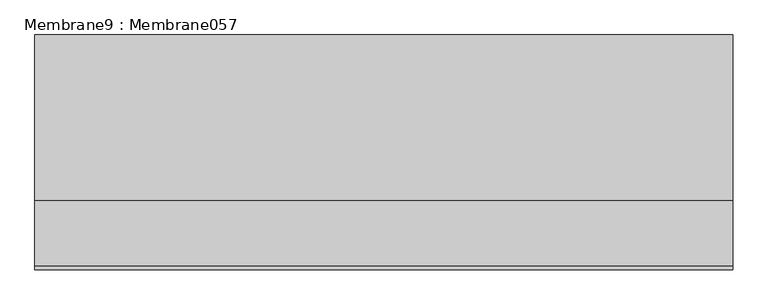
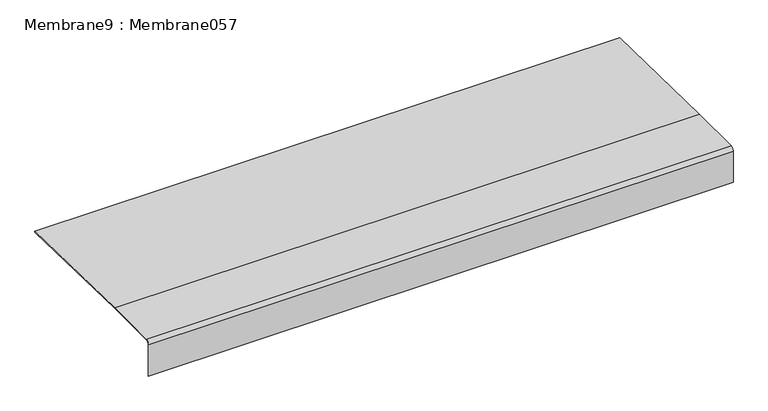
"""IFC4 building model written with IfcOpenShell, lengths in millimetres: proxy geometry, Membrane9 : Membrane057."""

import ifcopenshell
import ifcopenshell.guid

model = None  # the IFC model being written
_history = None  # IfcOwnerHistory: only IFC2X3 demands one
_inside = {}  # id of a spatial element -> (the spatial element, [elements in it])
_under = {}  # id of a project, library or spatial element -> (it, [spatial elements below it])
_declared = {}  # id of a project -> (the project, [libraries it declares])
_typed = {}  # id of a type object -> (the type object, [elements of that type])
_made_of = {}  # id of a material, layer set ... -> (it, [elements and type objects made of it])


def new_model(schema):
    """Start an empty IFC model of exactly this schema.

    Asked for "IFC4X3", IfcOpenShell would pick the latest addendum, in which some entities
    have other attributes; the version numbers below select the first issue.
    IFC2X3 requires an IfcOwnerHistory on every rooted entity: one is made here for all.
    """
    global model, _history
    if schema == "IFC4X3":
        model = ifcopenshell.file(schema_version=(4, 3, 0, 0))
    else:
        model = ifcopenshell.file(schema=schema)
    _inside.clear()
    _under.clear()
    _declared.clear()
    _typed.clear()
    _made_of.clear()
    _history = None
    if model.schema == "IFC2X3":
        org = make("IfcOrganization", Name="unknown")
        user = make(
            "IfcPersonAndOrganization",
            ThePerson=make("IfcPerson", FamilyName="unknown"),
            TheOrganization=org,
        )
        app = make(
            "IfcApplication",
            ApplicationDeveloper=org,
            Version="unknown",
            ApplicationFullName="unknown",
            ApplicationIdentifier="unknown",
        )
        _history = make(
            "IfcOwnerHistory",
            OwningUser=user,
            OwningApplication=app,
            ChangeAction="ADDED",
            CreationDate=0,
        )
    return model


def make(cls, **values):
    """One entity of the class cls with the attributes given. An attribute that is None is left unset."""
    return model.create_entity(
        cls, **{name: value for name, value in values.items() if value is not None}
    )


def rooted(cls, **values):
    """An entity with a GlobalId (a new one), such as an element, a storey or a relation."""
    return make(cls, GlobalId=ifcopenshell.guid.new(), OwnerHistory=_history, **values)


def si_unit(unit_type, name, prefix=None):
    """IfcSIUnit, for example si_unit("LENGTHUNIT", "METRE", prefix="MILLI")."""
    return make("IfcSIUnit", UnitType=unit_type, Prefix=prefix, Name=name)


def assignment(units):
    """IfcUnitAssignment: the units of a project."""
    return None if units is None else make("IfcUnitAssignment", Units=units)


def point(xyz):
    """IfcCartesianPoint."""
    return None if xyz is None else make("IfcCartesianPoint", Coordinates=xyz)


def direction(xyz):
    """IfcDirection."""
    return None if xyz is None else make("IfcDirection", DirectionRatios=xyz)


def frame(location, z_axis=None, x_axis=None):
    """IfcAxis2Placement3D, a coordinate frame: its origin and axes. An axis left out is left unset."""
    return make(
        "IfcAxis2Placement3D",
        Location=point(location),
        Axis=direction(z_axis),
        RefDirection=direction(x_axis),
    )


def frame_2d(location, x_axis=None):
    """IfcAxis2Placement2D, a coordinate frame in the plane: its origin and x axis."""
    return make(
        "IfcAxis2Placement2D", Location=point(location), RefDirection=direction(x_axis)
    )


def origin():
    """The frame at (0, 0, 0) with its axes left unset."""
    return frame((0.0, 0.0, 0.0))


def place(relative_to, where):
    """IfcLocalPlacement: puts the frame where relative to a parent placement (None: the world)."""
    return make(
        "IfcLocalPlacement", PlacementRelTo=relative_to, RelativePlacement=where
    )


def context(
    kind, dimensions, precision=None, world=None, true_north=None, identifier=None
):
    """IfcGeometricRepresentationContext, for example the 3D "Model" context."""
    return make(
        "IfcGeometricRepresentationContext",
        ContextIdentifier=identifier,
        ContextType=kind,
        CoordinateSpaceDimension=dimensions,
        Precision=precision,
        WorldCoordinateSystem=world,
        TrueNorth=true_north,
    )


def project(units=None, contexts=None):
    """IfcProject with its units and contexts."""
    return rooted(
        "IfcProject",
        Name="project",
        RepresentationContexts=contexts,
        UnitsInContext=assignment(units),
    )


def spatial(cls, under=None, at=None, **own):
    """A site, building, storey or space (cls), placed at a placement, below another one or the project."""
    s = rooted(cls, ObjectPlacement=at, **own)
    if under is not None:
        _under.setdefault(under.id(), (under, []))[1].append(s)
    return s


def polyline(points):
    """IfcPolyline through the points."""
    return make("IfcPolyline", Points=[point(p) for p in points])


def circle_curve(where, radius):
    """IfcCircle in the frame where."""
    return make("IfcCircle", Position=where, Radius=radius)


def trimmed(basis, trim1, trim2, sense, master):
    """IfcTrimmedCurve: the piece of a basis curve between two trims."""
    return make(
        "IfcTrimmedCurve",
        BasisCurve=basis,
        Trim1=trim1,
        Trim2=trim2,
        SenseAgreement=sense,
        MasterRepresentation=master,
    )


def segment(curve, same_sense, transition):
    """IfcCompositeCurveSegment."""
    return make(
        "IfcCompositeCurveSegment",
        Transition=transition,
        SameSense=same_sense,
        ParentCurve=curve,
    )


def composite_curve(segments, self_intersect=None):
    """IfcCompositeCurve: segments joined end to end."""
    return make("IfcCompositeCurve", Segments=segments, SelfIntersect=self_intersect)


def outline(outer, holes=None, kind="AREA"):
    """IfcArbitraryClosedProfileDef: a profile drawn as a closed curve; with holes, ...WithVoids."""
    if holes is None:
        return make("IfcArbitraryClosedProfileDef", ProfileType=kind, OuterCurve=outer)
    return make(
        "IfcArbitraryProfileDefWithVoids",
        ProfileType=kind,
        OuterCurve=outer,
        InnerCurves=holes,
    )


def extrude(swept, where, along, depth):
    """IfcExtrudedAreaSolid: the profile swept, set in the frame where, extruded along a direction by depth."""
    return make(
        "IfcExtrudedAreaSolid",
        SweptArea=swept,
        Position=where,
        ExtrudedDirection=direction(along),
        Depth=depth,
    )


def shape(context_of_items, identifier, shape_type, items):
    """IfcShapeRepresentation: the items that make up one representation, for example the "Body"."""
    return make(
        "IfcShapeRepresentation",
        ContextOfItems=context_of_items,
        RepresentationIdentifier=identifier,
        RepresentationType=shape_type,
        Items=items,
    )


def source(mapping_origin, context_of_items, identifier, shape_type, items):
    """IfcRepresentationMap: a shape defined once, which mapped items show again and again."""
    return make(
        "IfcRepresentationMap",
        MappingOrigin=mapping_origin,
        MappedRepresentation=shape(context_of_items, identifier, shape_type, items),
    )


def transform(
    local_origin,
    x_axis=None,
    y_axis=None,
    z_axis=None,
    scale=None,
    scale2=None,
    scale3=None,
    uniform=True,
):
    """IfcCartesianTransformationOperator3D, or its non-uniform kind. x_axis, y_axis, z_axis: its Axis1, 2, 3."""
    if uniform:
        return make(
            "IfcCartesianTransformationOperator3D",
            Axis1=direction(x_axis),
            Axis2=direction(y_axis),
            LocalOrigin=point(local_origin),
            Scale=scale,
            Axis3=direction(z_axis),
        )
    return make(
        "IfcCartesianTransformationOperator3DnonUniform",
        Axis1=direction(x_axis),
        Axis2=direction(y_axis),
        LocalOrigin=point(local_origin),
        Scale=scale,
        Axis3=direction(z_axis),
        Scale2=scale2,
        Scale3=scale3,
    )


def mapped(mapping_source, mapping_target):
    """IfcMappedItem: shows the shape of a source again, moved by a transform."""
    return make(
        "IfcMappedItem", MappingSource=mapping_source, MappingTarget=mapping_target
    )


def made_of(thing, what):
    """Note that an element or type object is made of a material, layer set ...; save() writes the relation."""
    if what is not None:
        _made_of.setdefault(what.id(), (what, []))[1].append(thing)
    return thing


def element(
    cls,
    number,
    at=None,
    inside=None,
    cuts=None,
    type_object=None,
    material=None,
    context=None,
    identifier="Body",
    shape_type=None,
    held_by="IfcProductDefinitionShape",
    body=None,
    shapes=None,
    **own,
):
    """One element of the class cls, such as IfcWall. Its Tag is "e" and its number.

    at: its placement. inside: the storey or other place that contains it. cuts: it is an
    opening in that element (IfcRelVoidsElement). A single representation is given by context,
    identifier, shape_type and body (its items); several are given by shapes. held_by: the class
    of the entity that holds the representations. save() writes the other relations.
    """
    e = rooted(cls, Tag="e%d" % number, ObjectPlacement=at, **own)
    if body is not None:
        shapes = [shape(context, identifier, shape_type, body)]
    if shapes is not None:
        e.Representation = make(held_by, Representations=shapes)
    if inside is not None:
        _inside.setdefault(inside.id(), (inside, []))[1].append(e)
    if cuts is not None:
        rooted(
            "IfcRelVoidsElement", RelatingBuildingElement=cuts, RelatedOpeningElement=e
        )
    if type_object is not None:
        _typed.setdefault(type_object.id(), (type_object, []))[1].append(e)
    return made_of(e, material)


def aggregate(whole, parts):
    """IfcRelAggregates: a whole, such as a stair, and the parts it consists of."""
    return rooted("IfcRelAggregates", RelatingObject=whole, RelatedObjects=parts)


def save(model, path):
    """Write the relations noted so far, then the file.

    IfcRelAggregates (storeys below a building ...), IfcRelContainedInSpatialStructure (elements
    in a storey), IfcRelDefinesByType, IfcRelAssociatesMaterial and IfcRelDeclares: one each for
    every whole, place, type object, material and project.
    """
    for whole, parts in _under.values():
        aggregate(whole, parts)
    for where, things in _inside.values():
        rooted(
            "IfcRelContainedInSpatialStructure",
            RelatedElements=things,
            RelatingStructure=where,
        )
    for kind, things in _typed.values():
        rooted("IfcRelDefinesByType", RelatedObjects=things, RelatingType=kind)
    for what, things in _made_of.values():
        rooted("IfcRelAssociatesMaterial", RelatedObjects=things, RelatingMaterial=what)
    for by, libraries in _declared.values():
        rooted("IfcRelDeclares", RelatingContext=by, RelatedDefinitions=libraries)
    model.write(path)


def membrane9_membrane057_6ca42c2d(model_context):
    return source(origin(), model_context, "Body", "SweptSolid", [
        extrude(outline(composite_curve([segment(polyline([(-5547.5899524, 40106.229319), (-5549.5899524, 40106.229319), (-5549.5899524, 40219.8534812)]), True, "CONTINUOUS"), segment(trimmed(circle_curve(frame_2d((-5537.5899524, 40219.8534812)), 12.0), [point((-5549.5899524, 40219.8534812))], [point((-5537.5899524, 40231.8534812))], False, "CARTESIAN"), True, "CONTINUOUS"), segment(polyline([(-5537.5899524, 40231.8534812), (-5350.1524727, 40231.8534812), (-4876.5591046, 40221.0182087), (-4876.6048503, 40219.0187319), (-5350.1753483, 40229.8534812), (-5537.5899524, 40229.8534812)]), True, "CONTINUOUS"), segment(trimmed(circle_curve(frame_2d((-5537.5899524, 40219.8534812)), 10.0), [point((-5537.5899524, 40229.8534812))], [point((-5547.5899524, 40219.8534812))], True, "CARTESIAN"), True, "CONTINUOUS"), segment(polyline([(-5547.5899524, 40219.8534812), (-5547.5899524, 40106.229319)]), True, "CONTINUOUS")], self_intersect=False)), frame((12383.0178845, 0.0, 0.0), z_axis=(1.0, 0.0, 0.0), x_axis=(0.0, 1.0, 0.0)), (0.0, 0.0, 1.0), 2000.0),
    ])


if __name__ == "__main__":
    model = new_model("IFC4")
    model_context = context("Model", 3, world=origin())
    ifc_project = project(units=[si_unit("LENGTHUNIT", "METRE", prefix="MILLI")], contexts=[model_context])
    site = spatial("IfcSite", under=ifc_project)
    building = spatial("IfcBuilding", under=site)
    placement = place(None, origin())
    membrane9_membrane057_shape = membrane9_membrane057_6ca42c2d(model_context)
    element("IfcBuildingElementProxy", 1, Name="Membrane9 : Membrane057", ObjectType="Membrane9 : Membrane057", at=placement, inside=building, context=model_context, shape_type="MappedRepresentation", body=[
        mapped(membrane9_membrane057_shape, transform((0.0, 0.0, 0.0), x_axis=(1.0, 0.0, 0.0), y_axis=(0.0, 1.0, 0.0), z_axis=(0.0, 0.0, 1.0))),
    ])
    save(model, "model.ifc")

# Revit data of these elements
# Type "Membrane9 : Membrane057"
#   NameOverride = "Membrane057"
# Element 1 (IfcBuildingElementProxy, "Membrane9 : Membrane057")
#   Materials on its faces: "THREE PLY BUILT UP ROOF MEMBRANE"
# Materials
#   "THREE PLY BUILT UP ROOF MEMBRANE": class "Unassigned", colour RGB 63 63 63, transparency 0
